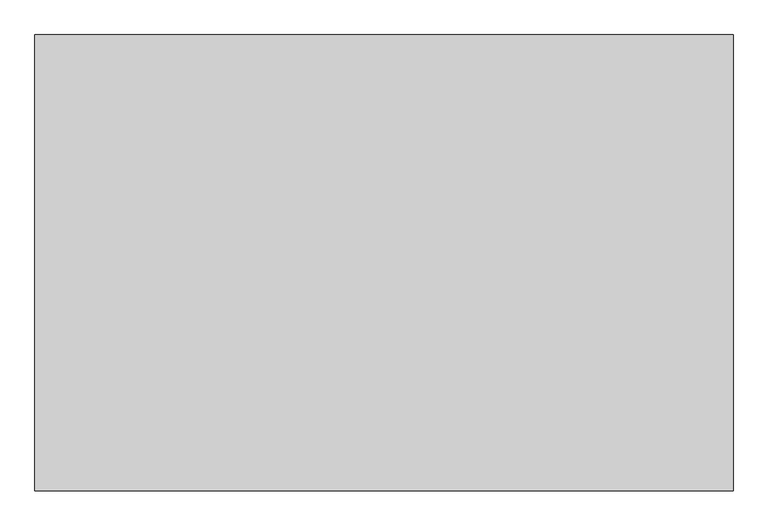
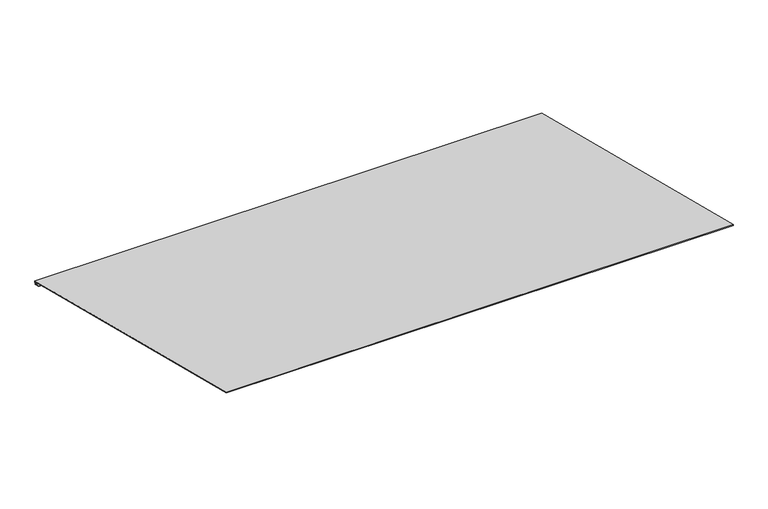
"""IFC4 building model written with IfcOpenShell, lengths in millimetres: proxy geometry, Gutter @ Roof001 3953 : Gutter @ Roof001 3953."""

import ifcopenshell
import ifcopenshell.guid

model = None  # the IFC model being written
_history = None  # IfcOwnerHistory: only IFC2X3 demands one
_inside = {}  # id of a spatial element -> (the spatial element, [elements in it])
_under = {}  # id of a project, library or spatial element -> (it, [spatial elements below it])
_declared = {}  # id of a project -> (the project, [libraries it declares])
_typed = {}  # id of a type object -> (the type object, [elements of that type])
_made_of = {}  # id of a material, layer set ... -> (it, [elements and type objects made of it])


def new_model(schema):
    """Start an empty IFC model of exactly this schema.

    Asked for "IFC4X3", IfcOpenShell would pick the latest addendum, in which some entities
    have other attributes; the version numbers below select the first issue.
    IFC2X3 requires an IfcOwnerHistory on every rooted entity: one is made here for all.
    """
    global model, _history
    if schema == "IFC4X3":
        model = ifcopenshell.file(schema_version=(4, 3, 0, 0))
    else:
        model = ifcopenshell.file(schema=schema)
    _inside.clear()
    _under.clear()
    _declared.clear()
    _typed.clear()
    _made_of.clear()
    _history = None
    if model.schema == "IFC2X3":
        org = make("IfcOrganization", Name="unknown")
        user = make(
            "IfcPersonAndOrganization",
            ThePerson=make("IfcPerson", FamilyName="unknown"),
            TheOrganization=org,
        )
        app = make(
            "IfcApplication",
            ApplicationDeveloper=org,
            Version="unknown",
            ApplicationFullName="unknown",
            ApplicationIdentifier="unknown",
        )
        _history = make(
            "IfcOwnerHistory",
            OwningUser=user,
            OwningApplication=app,
            ChangeAction="ADDED",
            CreationDate=0,
        )
    return model


def make(cls, **values):
    """One entity of the class cls with the attributes given. An attribute that is None is left unset."""
    return model.create_entity(
        cls, **{name: value for name, value in values.items() if value is not None}
    )


def rooted(cls, **values):
    """An entity with a GlobalId (a new one), such as an element, a storey or a relation."""
    return make(cls, GlobalId=ifcopenshell.guid.new(), OwnerHistory=_history, **values)


def si_unit(unit_type, name, prefix=None):
    """IfcSIUnit, for example si_unit("LENGTHUNIT", "METRE", prefix="MILLI")."""
    return make("IfcSIUnit", UnitType=unit_type, Prefix=prefix, Name=name)


def assignment(units):
    """IfcUnitAssignment: the units of a project."""
    return None if units is None else make("IfcUnitAssignment", Units=units)


def point(xyz):
    """IfcCartesianPoint."""
    return None if xyz is None else make("IfcCartesianPoint", Coordinates=xyz)


def direction(xyz):
    """IfcDirection."""
    return None if xyz is None else make("IfcDirection", DirectionRatios=xyz)


def frame(location, z_axis=None, x_axis=None):
    """IfcAxis2Placement3D, a coordinate frame: its origin and axes. An axis left out is left unset."""
    return make(
        "IfcAxis2Placement3D",
        Location=point(location),
        Axis=direction(z_axis),
        RefDirection=direction(x_axis),
    )


def origin():
    """The frame at (0, 0, 0) with its axes left unset."""
    return frame((0.0, 0.0, 0.0))


def place(relative_to, where):
    """IfcLocalPlacement: puts the frame where relative to a parent placement (None: the world)."""
    return make(
        "IfcLocalPlacement", PlacementRelTo=relative_to, RelativePlacement=where
    )


def context(
    kind, dimensions, precision=None, world=None, true_north=None, identifier=None
):
    """IfcGeometricRepresentationContext, for example the 3D "Model" context."""
    return make(
        "IfcGeometricRepresentationContext",
        ContextIdentifier=identifier,
        ContextType=kind,
        CoordinateSpaceDimension=dimensions,
        Precision=precision,
        WorldCoordinateSystem=world,
        TrueNorth=true_north,
    )


def project(units=None, contexts=None):
    """IfcProject with its units and contexts."""
    return rooted(
        "IfcProject",
        Name="project",
        RepresentationContexts=contexts,
        UnitsInContext=assignment(units),
    )


def spatial(cls, under=None, at=None, **own):
    """A site, building, storey or space (cls), placed at a placement, below another one or the project."""
    s = rooted(cls, ObjectPlacement=at, **own)
    if under is not None:
        _under.setdefault(under.id(), (under, []))[1].append(s)
    return s


def polyline(points):
    """IfcPolyline through the points."""
    return make("IfcPolyline", Points=[point(p) for p in points])


def outline(outer, holes=None, kind="AREA"):
    """IfcArbitraryClosedProfileDef: a profile drawn as a closed curve; with holes, ...WithVoids."""
    if holes is None:
        return make("IfcArbitraryClosedProfileDef", ProfileType=kind, OuterCurve=outer)
    return make(
        "IfcArbitraryProfileDefWithVoids",
        ProfileType=kind,
        OuterCurve=outer,
        InnerCurves=holes,
    )


def extrude(swept, where, along, depth):
    """IfcExtrudedAreaSolid: the profile swept, set in the frame where, extruded along a direction by depth."""
    return make(
        "IfcExtrudedAreaSolid",
        SweptArea=swept,
        Position=where,
        ExtrudedDirection=direction(along),
        Depth=depth,
    )


def shape(context_of_items, identifier, shape_type, items):
    """IfcShapeRepresentation: the items that make up one representation, for example the "Body"."""
    return make(
        "IfcShapeRepresentation",
        ContextOfItems=context_of_items,
        RepresentationIdentifier=identifier,
        RepresentationType=shape_type,
        Items=items,
    )


def source(mapping_origin, context_of_items, identifier, shape_type, items):
    """IfcRepresentationMap: a shape defined once, which mapped items show again and again."""
    return make(
        "IfcRepresentationMap",
        MappingOrigin=mapping_origin,
        MappedRepresentation=shape(context_of_items, identifier, shape_type, items),
    )


def transform(
    local_origin,
    x_axis=None,
    y_axis=None,
    z_axis=None,
    scale=None,
    scale2=None,
    scale3=None,
    uniform=True,
):
    """IfcCartesianTransformationOperator3D, or its non-uniform kind. x_axis, y_axis, z_axis: its Axis1, 2, 3."""
    if uniform:
        return make(
            "IfcCartesianTransformationOperator3D",
            Axis1=direction(x_axis),
            Axis2=direction(y_axis),
            LocalOrigin=point(local_origin),
            Scale=scale,
            Axis3=direction(z_axis),
        )
    return make(
        "IfcCartesianTransformationOperator3DnonUniform",
        Axis1=direction(x_axis),
        Axis2=direction(y_axis),
        LocalOrigin=point(local_origin),
        Scale=scale,
        Axis3=direction(z_axis),
        Scale2=scale2,
        Scale3=scale3,
    )


def mapped(mapping_source, mapping_target):
    """IfcMappedItem: shows the shape of a source again, moved by a transform."""
    return make(
        "IfcMappedItem", MappingSource=mapping_source, MappingTarget=mapping_target
    )


def made_of(thing, what):
    """Note that an element or type object is made of a material, layer set ...; save() writes the relation."""
    if what is not None:
        _made_of.setdefault(what.id(), (what, []))[1].append(thing)
    return thing


def element(
    cls,
    number,
    at=None,
    inside=None,
    cuts=None,
    type_object=None,
    material=None,
    context=None,
    identifier="Body",
    shape_type=None,
    held_by="IfcProductDefinitionShape",
    body=None,
    shapes=None,
    **own,
):
    """One element of the class cls, such as IfcWall. Its Tag is "e" and its number.

    at: its placement. inside: the storey or other place that contains it. cuts: it is an
    opening in that element (IfcRelVoidsElement). A single representation is given by context,
    identifier, shape_type and body (its items); several are given by shapes. held_by: the class
    of the entity that holds the representations. save() writes the other relations.
    """
    e = rooted(cls, Tag="e%d" % number, ObjectPlacement=at, **own)
    if body is not None:
        shapes = [shape(context, identifier, shape_type, body)]
    if shapes is not None:
        e.Representation = make(held_by, Representations=shapes)
    if inside is not None:
        _inside.setdefault(inside.id(), (inside, []))[1].append(e)
    if cuts is not None:
        rooted(
            "IfcRelVoidsElement", RelatingBuildingElement=cuts, RelatedOpeningElement=e
        )
    if type_object is not None:
        _typed.setdefault(type_object.id(), (type_object, []))[1].append(e)
    return made_of(e, material)


def aggregate(whole, parts):
    """IfcRelAggregates: a whole, such as a stair, and the parts it consists of."""
    return rooted("IfcRelAggregates", RelatingObject=whole, RelatedObjects=parts)


def save(model, path):
    """Write the relations noted so far, then the file.

    IfcRelAggregates (storeys below a building ...), IfcRelContainedInSpatialStructure (elements
    in a storey), IfcRelDefinesByType, IfcRelAssociatesMaterial and IfcRelDeclares: one each for
    every whole, place, type object, material and project.
    """
    for whole, parts in _under.values():
        aggregate(whole, parts)
    for where, things in _inside.values():
        rooted(
            "IfcRelContainedInSpatialStructure",
            RelatedElements=things,
            RelatingStructure=where,
        )
    for kind, things in _typed.values():
        rooted("IfcRelDefinesByType", RelatedObjects=things, RelatingType=kind)
    for what, things in _made_of.values():
        rooted("IfcRelAssociatesMaterial", RelatedObjects=things, RelatingMaterial=what)
    for by, libraries in _declared.values():
        rooted("IfcRelDeclares", RelatingContext=by, RelatedDefinitions=libraries)
    model.write(path)


def generic_models_4c0e396c(model_context):
    return source(origin(), model_context, "Body", "SweptSolid", [
        extrude(outline(polyline([(3064.132137, 41849.8246764), (4371.4558626, 41522.9928253), (4368.0267643, 41509.2764322), (4346.0295733, 41514.9618766), (4346.6651806, 41517.4210642), (4366.183559, 41512.3762993), (4368.3756601, 41521.1447038), (3064.132137, 41847.2055846), (3064.132137, 41849.8246764)])), frame((255.0171875, 0.0, 0.0), z_axis=(1.0, 0.0, 0.0), x_axis=(0.0, 1.0, 0.0)), (0.0, 0.0, 1.0), 1999.85),
    ])


if __name__ == "__main__":
    model = new_model("IFC4")
    model_context = context("Model", 3, world=origin())
    ifc_project = project(units=[si_unit("LENGTHUNIT", "METRE", prefix="MILLI")], contexts=[model_context])
    site = spatial("IfcSite", under=ifc_project)
    building = spatial("IfcBuilding", under=site)
    placement = place(None, origin())
    generic_models_shape = generic_models_4c0e396c(model_context)
    element("IfcBuildingElementProxy", 1, Name="Gutter @ Roof001 3953 : Gutter @ Roof001 3953", ObjectType="Gutter @ Roof001 3953 : Gutter @ Roof001 3953", at=placement, inside=building, context=model_context, shape_type="MappedRepresentation", body=[
        mapped(generic_models_shape, transform((0.0, 0.0, 0.0), x_axis=(1.0, 0.0, 0.0), y_axis=(0.0, 1.0, 0.0), z_axis=(0.0, 0.0, 1.0))),
    ])
    save(model, "model.ifc")

# Revit data of these elements
# Type "Gutter @ Roof001 3953 : Gutter @ Roof001 3953"
#   NameOverride = "Gutter @ Roof001"
# Element 1 (IfcBuildingElementProxy, "Gutter @ Roof001 3953 : Gutter @ Roof001 3953")
#   Materials on its faces: "CONT. SEAMLESS 16 GA COPPER BRAKE METAL GUTTER"
# Materials
#   "CONT. SEAMLESS 16 GA COPPER BRAKE METAL GUTTER": class "Unassigned", colour RGB 128 128 128, transparency 0
